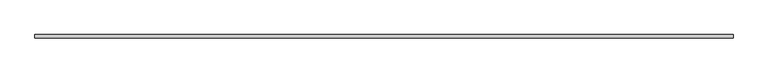
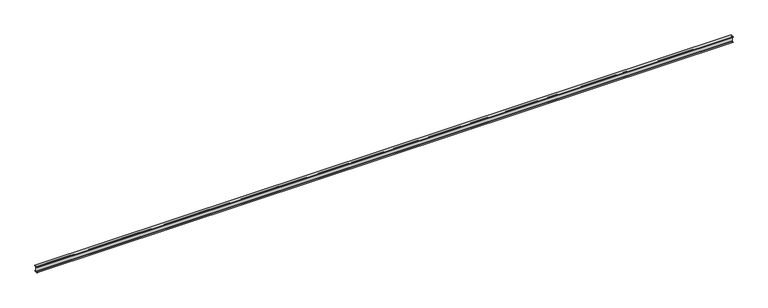
"""IFC4 building model written with IfcOpenShell, lengths in millimetres: beam geometry, Steel Framing_H_KS : H_SB_AR_S02_H-488x300x11x18_CRG1."""

from ifc_helpers import new_model, si_unit, point, frame, frame_2d, origin, place, context, project, spatial, polyline, circle_curve, trimmed, segment, composite_curve, outline, extrude, source, transform, mapped, element, save


def beam_70e5a2de(model_context):
    return source(origin(), model_context, "Body", "SweptSolid", [
        extrude(outline(composite_curve([segment(polyline([(150.0, -226.0), (150.0, -244.0), (-150.0, -244.0), (-150.0, -226.0), (-31.5, -226.0)]), True, "CONTINUOUS"), segment(trimmed(circle_curve(frame_2d((-31.5, -200.0)), 26.0), [point((-31.5, -226.0))], [point((-5.5, -200.0))], True, "CARTESIAN"), True, "CONTINUOUS"), segment(polyline([(-5.5, -200.0), (-5.5, 200.0)]), True, "CONTINUOUS"), segment(trimmed(circle_curve(frame_2d((-31.5, 200.0)), 26.0), [point((-5.5, 200.0))], [point((-31.5, 226.0))], True, "CARTESIAN"), True, "CONTINUOUS"), segment(polyline([(-31.5, 226.0), (-150.0, 226.0), (-150.0, 244.0), (150.0, 244.0), (150.0, 226.0), (31.5, 226.0)]), True, "CONTINUOUS"), segment(trimmed(circle_curve(frame_2d((31.5, 200.0)), 26.0), [point((31.5, 226.0))], [point((5.5, 200.0))], True, "CARTESIAN"), True, "CONTINUOUS"), segment(polyline([(5.5, 200.0), (5.5, -200.0)]), True, "CONTINUOUS"), segment(trimmed(circle_curve(frame_2d((31.5, -200.0)), 26.0), [point((5.5, -200.0))], [point((31.5, -226.0))], True, "CARTESIAN"), True, "CONTINUOUS"), segment(polyline([(31.5, -226.0), (150.0, -226.0)]), True, "CONTINUOUS")], self_intersect=False)), frame((-30000.0, 0.0, 0.0), z_axis=(1.0, 0.0, 0.0), x_axis=(0.0, 1.0, 0.0)), (0.0, 0.0, 1.0), 60000.0),
    ])


if __name__ == "__main__":
    model = new_model("IFC4")
    model_context = context("Model", 3, world=origin())
    ifc_project = project(units=[si_unit("LENGTHUNIT", "METRE", prefix="MILLI")], contexts=[model_context])
    site = spatial("IfcSite", under=ifc_project)
    building = spatial("IfcBuilding", under=site)
    placement = place(None, origin())
    beam_shape = beam_70e5a2de(model_context)
    element("IfcBeam", 1, ObjectType="Steel Framing_H_KS : H_SB_AR_S02_H-488x300x11x18_CRG1", at=placement, inside=building, context=model_context, shape_type="MappedRepresentation", body=[
        mapped(beam_shape, transform((0.0, 0.0, 0.0), x_axis=(1.0, 0.0, 0.0), y_axis=(0.0, 1.0, 0.0), z_axis=(0.0, 0.0, 1.0))),
    ])
    save(model, "model.ifc")

# Revit data of these elements
# Type "Steel Framing_H_KS : H_SB_AR_S02_H-488x300x11x18_CRG1"
#   Type Comments = "MAIN"
#   Type Mark = "CRG1"
#   H_SectionID = "H-488x300x11x18"
#   H_Ratio for Additional Steel Plate = 0.2
#   Width = 30.0 cm
#   Web Thickness = 1.1 cm
#   Web Fillet = 2.6 cm
#   Warping Constant = 4470000.0 cm⁶
#   Torsional Moment of Inertia = 137.492 cm⁴
#   Section Area = 163.5 cm²
#   Plastic Modulus weak axis = 830.0 cm³
#   Plastic Modulus strong axis = 3230.0 cm³
#   Perimeter = 2.11 m²/m
#   Nominal Weight = 128.00 kgf/m
#   Moment of Inertia weak axis = 8110.00 cm⁴
#   Moment of Inertia strong axis = 71000.00 cm⁴
#   Height = 48.8 cm
#   Flange Thickness = 1.8 cm
#   Elastic Modulus weak axis = 541.0 cm³
#   Elastic Modulus strong axis = 2910.0 cm³
#   Centroid Vertical = 24.4 cm
#   Centroid Horizontal = 15.0 cm
#   Bolt Spacing = 8.89 cm
#   Length [instance default] = 1500 mm
#   Structural Material [instance default] = Steel, 45-345
#   Section Name Key = ""
#   Assembly Code = ""
# Element 1 (IfcBeam, "Steel Framing_H_KS : H_SB_AR_S02_H-488x300x11x18_CRG1")
#   Materials on its faces: "Steel, 45-345"
# Materials
#   "Steel, 45-345": class "Metal", colour RGB 189 187 185, transparency 0, Description = "Steel 345 MPa", Cost = 0
